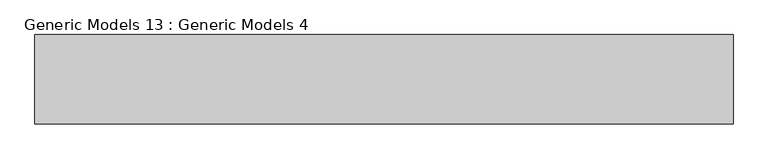
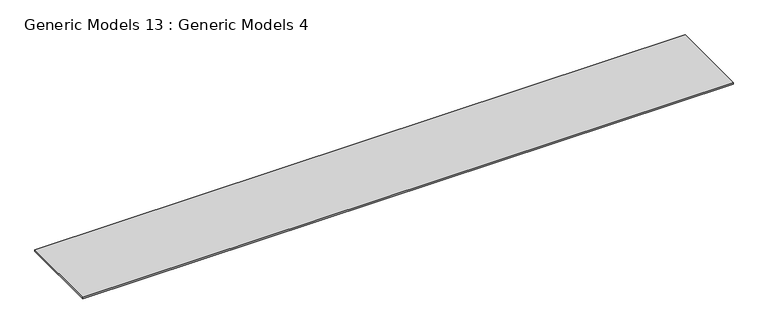
"""IFC4 building model written with IfcOpenShell, lengths in millimetres: proxy geometry, Generic Models 13 : Generic Models 4."""

from ifc_helpers import new_model, si_unit, frame, origin, place, context, project, spatial, polyline, outline, extrude, source, transform, mapped, element, save


def generic_models_13_generic_models_4_e7f441bd(model_context):
    return source(origin(), model_context, "Body", "SweptSolid", [
        extrude(outline(polyline([(8386.8578684, -6080.7311742), (8386.8578684, -6871.9053756), (2196.9263704, -6871.9053756), (2196.9263704, -6080.7311742), (8386.8578684, -6080.7311742)])), frame((0.0, 0.0, 126355.8662959), z_axis=(0.0, 0.0, 1.0), x_axis=(1.0, 0.0, 0.0)), (0.0, 0.0, 1.0), 15.875),
    ])


if __name__ == "__main__":
    model = new_model("IFC4")
    model_context = context("Model", 3, world=origin())
    ifc_project = project(units=[si_unit("LENGTHUNIT", "METRE", prefix="MILLI")], contexts=[model_context])
    site = spatial("IfcSite", under=ifc_project)
    building = spatial("IfcBuilding", under=site)
    placement = place(None, origin())
    generic_models_13_generic_models_4_shape = generic_models_13_generic_models_4_e7f441bd(model_context)
    element("IfcBuildingElementProxy", 1, Name="Generic Models 13 : Generic Models 4", ObjectType="Generic Models 13 : Generic Models 4", at=placement, inside=building, context=model_context, shape_type="MappedRepresentation", body=[
        mapped(generic_models_13_generic_models_4_shape, transform((0.0, 0.0, 0.0), x_axis=(1.0, 0.0, 0.0), y_axis=(0.0, 1.0, 0.0), z_axis=(0.0, 0.0, 1.0))),
    ])
    save(model, "model.ifc")

# Revit data of these elements
# Element 1 (IfcBuildingElementProxy, "Generic Models 13 : Generic Models 4")
#   Materials on its faces: "_5/8\" DRYWALL"
# Materials
#   "_5/8\" DRYWALL": class "Generic", colour RGB 191 191 191, transparency 0, Cost = 0
